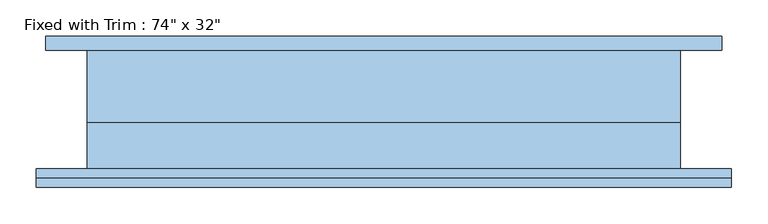
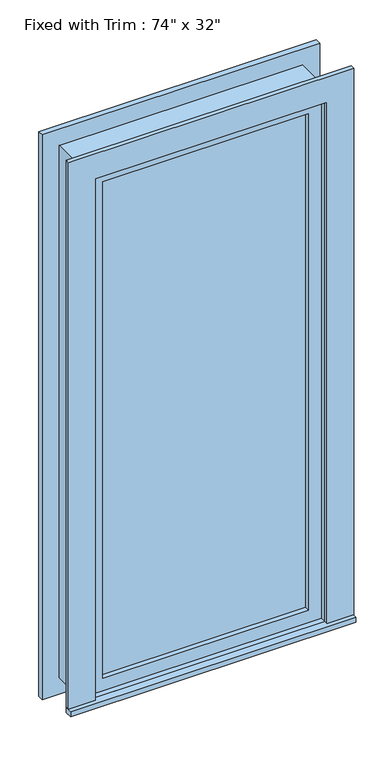
"""IFC4 building model written with IfcOpenShell, lengths in millimetres: window geometry."""

from ifc_helpers import new_model, si_unit, frame, origin, place, context, project, spatial, polyline, outline, extrude, source, transform, mapped, element, save


def window_4522221a(model_context):
    return source(origin(), model_context, "Body", "SweptSolid", [
        extrude(outline(polyline([(-514.35, -106.3625), (-514.35, -80.9625), (438.15, -80.9625), (438.15, -106.3625), (-514.35, -106.3625)])), frame((0.0, 0.0, 914.4), z_axis=(0.0, 0.0, 1.0), x_axis=(1.0, 0.0, 0.0)), (0.0, 0.0, 1.0), 19.05),
        extrude(outline(polyline([(2774.95, -425.45), (2774.95, 349.25), (933.45, 349.25), (933.45, 438.15), (2863.85, 438.15), (2863.85, -514.35), (933.45, -514.35), (933.45, -425.45), (2774.95, -425.45)])), frame((0.0, -93.6625, 0.0), z_axis=(0.0, 1.0, 0.0), x_axis=(0.0, 0.0, 1.0)), (0.0, 0.0, 1.0), 12.7),
        extrude(outline(polyline([(2851.15, 425.45), (2851.15, -501.65), (857.25, -501.65), (857.25, 425.45), (2851.15, 425.45)]), holes=[polyline([(2762.25, 336.55), (946.15, 336.55), (946.15, -412.75), (2762.25, -412.75), (2762.25, 336.55)])]), frame((0.0, 80.9625, 0.0), z_axis=(0.0, 1.0, 0.0), x_axis=(0.0, 0.0, 1.0)), (0.0, 0.0, 1.0), 19.05),
        extrude(outline(polyline([(304.8, -33.3375), (304.8, -46.0375), (-381.0, -46.0375), (-381.0, -33.3375), (304.8, -33.3375)])), frame((0.0, 0.0, 977.9), z_axis=(0.0, 0.0, 1.0), x_axis=(1.0, 0.0, 0.0)), (0.0, 0.0, 1.0), 1752.6),
        extrude(outline(polyline([(2774.95, -425.45), (933.45, -425.45), (933.45, 349.25), (2774.95, 349.25), (2774.95, -425.45)]), holes=[polyline([(2730.5, -381.0), (2730.5, 304.8), (977.9, 304.8), (977.9, -381.0), (2730.5, -381.0)])]), frame((0.0, -61.9125, 0.0), z_axis=(0.0, 1.0, 0.0), x_axis=(0.0, 0.0, 1.0)), (0.0, 0.0, 1.0), 44.45),
        extrude(outline(polyline([(2794.0, -444.5), (914.4, -444.5), (914.4, 368.3), (2794.0, 368.3), (2794.0, -444.5)]), holes=[polyline([(2762.25, -412.75), (2762.25, 336.55), (946.15, 336.55), (946.15, -412.75), (2762.25, -412.75)])]), frame((0.0, -17.4625, 0.0), z_axis=(0.0, 1.0, 0.0), x_axis=(0.0, 0.0, 1.0)), (0.0, 0.0, 1.0), 98.425),
        extrude(outline(polyline([(2794.0, 368.3), (2794.0, -444.5), (914.4, -444.5), (914.4, 368.3), (2794.0, 368.3)]), holes=[polyline([(2774.95, 349.25), (933.45, 349.25), (933.45, -425.45), (2774.95, -425.45), (2774.95, 349.25)])]), frame((0.0, -80.9625, 0.0), z_axis=(0.0, 1.0, 0.0), x_axis=(0.0, 0.0, 1.0)), (0.0, 0.0, 1.0), 63.5),
    ])


if __name__ == "__main__":
    model = new_model("IFC4")
    model_context = context("Model", 3, world=origin())
    ifc_project = project(units=[si_unit("LENGTHUNIT", "METRE", prefix="MILLI")], contexts=[model_context])
    site = spatial("IfcSite", under=ifc_project)
    building = spatial("IfcBuilding", under=site)
    placement = place(None, origin())
    window_shape = window_4522221a(model_context)
    element("IfcWindow", 1, ObjectType="Fixed with Trim : 74\" x 32\"", at=placement, inside=building, context=model_context, shape_type="MappedRepresentation", body=[
        mapped(window_shape, transform((0.0, 0.0, 0.0), x_axis=(1.0, 0.0, 0.0), y_axis=(0.0, 1.0, 0.0), z_axis=(0.0, 0.0, 1.0))),
    ])
    save(model, "model.ifc")

# Revit data of these elements
# Type "Fixed with Trim : 74\" x 32\""
#   Type Mark = "57"
#   COBie.Type.CreatedBy = "doug.wood@us.ibm.com"
#   COBie.Type.CreatedOn = "2016-04-14T02:07:26"
#   COBie.Type.Name = "Windows_Fixed with Trim_74\" x 32\"_57"
#   COBie.Type.Category = "23-30 20 17 11 : Fixed Windows"
#   COBie.Type.Description = "Fixed with Trim_74\" x 32\""
#   COBie.Type.Manufacturer = ""
#   COBie.Type.ModelNumber = ""
#   Construction Type Id = "GSP4R"
#   Assembly Code = "B2020100"
#   Analytic Construction = "1/8 in Pilkington single glazing"
#   COBie.Type.ReplacementCost = 0
#   Visual Light Transmittance = 0.9
#   Solar Heat Gain Coefficient = 0.78
#   Heat Transfer Coefficient (U) = 3.6886 W/(m²·K)
#   Height = 6' - 2"
#   Default Sill Height = 3' - 0"
#   Trim Projection - Ext. = 0' - 0 1/2"
#   Trim Projection - Int. = 0' - 0 3/4"
#   Trim Width - Exterior = 0' - 3 1/2"
#   Trim Width - Interior = 0' - 3 1/2"
#   Width = 2' - 8"
#   Window Inset = 0' - 0 3/4"
#   COBie.Type = no
#   Glass Pane Material = Glass
#   Sash Material = Sash - White
#   Trim Exterior Material = Trim - White
#   Trim Interior Material = Trim - White
#   Wall Closure = (empty or 0)
# Element 1 (IfcWindow, "Fixed with Trim : 74\" x 32\"")
#   Materials on its faces: "Sash - White", "Trim - White", "Glass"
# Materials
#   "Glass": class "Glass", colour RGB 0 128 192, transparency 0.75, Description = "Soda Lime Glass", Cost = 0
#   "Sash - White": class "Wood", colour RGB 255 255 255, transparency 0, Cost = 0
#   "Trim - White": class "Wood", colour RGB 255 255 255, transparency 0, Cost = 0
